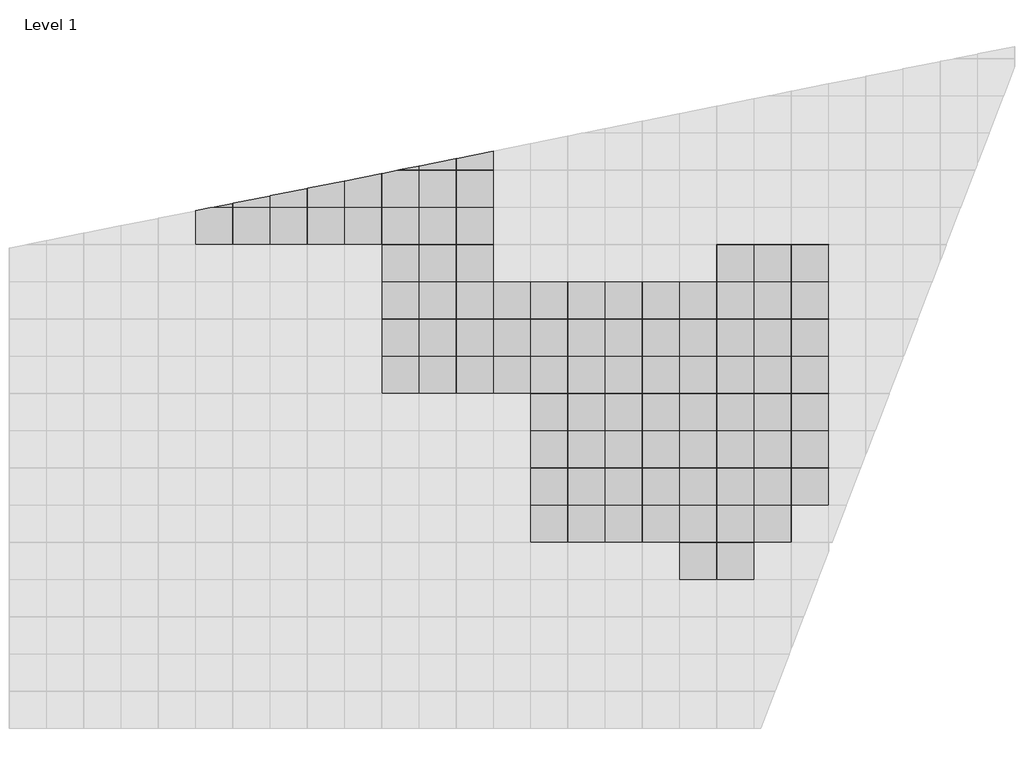
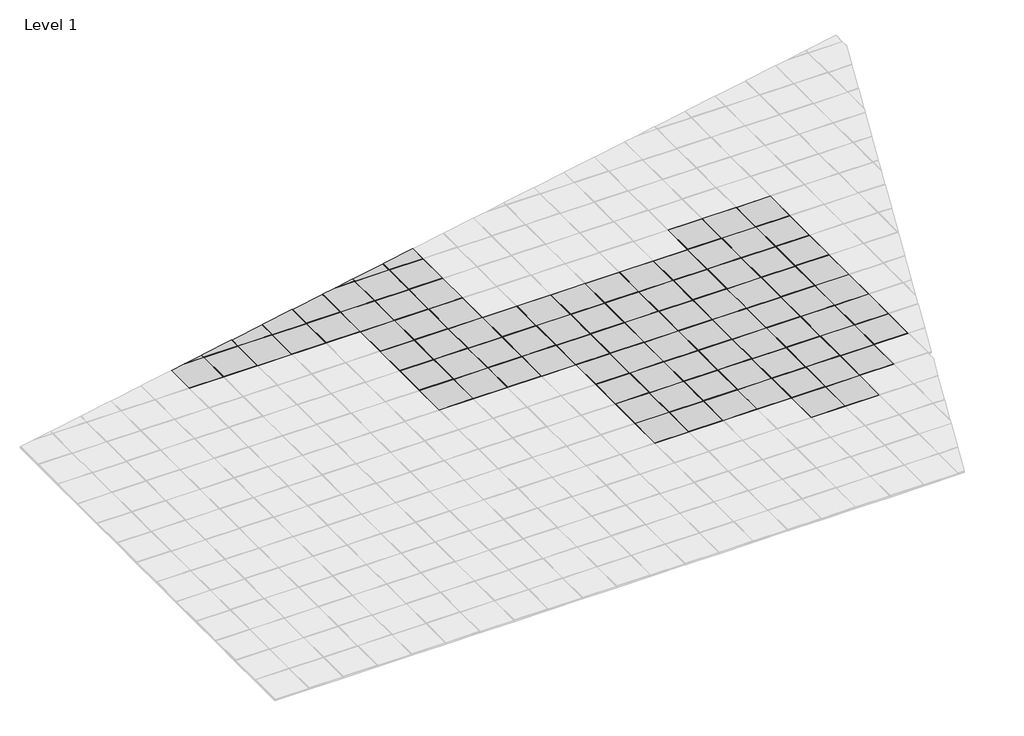
# One storey, part 6 of 18: 94 plates.
"""IFC4 building model written with IfcOpenShell, lengths in millimetres."""

import ifcopenshell
import ifcopenshell.guid

model = None  # the IFC model being written
_history = None  # IfcOwnerHistory: only IFC2X3 demands one
_inside = {}  # id of a spatial element -> (the spatial element, [elements in it])
_under = {}  # id of a project, library or spatial element -> (it, [spatial elements below it])
_declared = {}  # id of a project -> (the project, [libraries it declares])
_typed = {}  # id of a type object -> (the type object, [elements of that type])
_made_of = {}  # id of a material, layer set ... -> (it, [elements and type objects made of it])


def new_model(schema):
    """Start an empty IFC model of exactly this schema.

    Asked for "IFC4X3", IfcOpenShell would pick the latest addendum, in which some entities
    have other attributes; the version numbers below select the first issue.
    IFC2X3 requires an IfcOwnerHistory on every rooted entity: one is made here for all.
    """
    global model, _history
    if schema == "IFC4X3":
        model = ifcopenshell.file(schema_version=(4, 3, 0, 0))
    else:
        model = ifcopenshell.file(schema=schema)
    _inside.clear()
    _under.clear()
    _declared.clear()
    _typed.clear()
    _made_of.clear()
    _history = None
    if model.schema == "IFC2X3":
        org = make("IfcOrganization", Name="unknown")
        user = make(
            "IfcPersonAndOrganization",
            ThePerson=make("IfcPerson", FamilyName="unknown"),
            TheOrganization=org,
        )
        app = make(
            "IfcApplication",
            ApplicationDeveloper=org,
            Version="unknown",
            ApplicationFullName="unknown",
            ApplicationIdentifier="unknown",
        )
        _history = make(
            "IfcOwnerHistory",
            OwningUser=user,
            OwningApplication=app,
            ChangeAction="ADDED",
            CreationDate=0,
        )
    return model


def make(cls, **values):
    """One entity of the class cls with the attributes given. An attribute that is None is left unset."""
    return model.create_entity(
        cls, **{name: value for name, value in values.items() if value is not None}
    )


def rooted(cls, **values):
    """An entity with a GlobalId (a new one), such as an element, a storey or a relation."""
    return make(cls, GlobalId=ifcopenshell.guid.new(), OwnerHistory=_history, **values)


def si_unit(unit_type, name, prefix=None):
    """IfcSIUnit, for example si_unit("LENGTHUNIT", "METRE", prefix="MILLI")."""
    return make("IfcSIUnit", UnitType=unit_type, Prefix=prefix, Name=name)


def assignment(units):
    """IfcUnitAssignment: the units of a project."""
    return None if units is None else make("IfcUnitAssignment", Units=units)


def point(xyz):
    """IfcCartesianPoint."""
    return None if xyz is None else make("IfcCartesianPoint", Coordinates=xyz)


def direction(xyz):
    """IfcDirection."""
    return None if xyz is None else make("IfcDirection", DirectionRatios=xyz)


def frame(location, z_axis=None, x_axis=None):
    """IfcAxis2Placement3D, a coordinate frame: its origin and axes. An axis left out is left unset."""
    return make(
        "IfcAxis2Placement3D",
        Location=point(location),
        Axis=direction(z_axis),
        RefDirection=direction(x_axis),
    )


def origin():
    """The frame at (0, 0, 0) with its axes left unset."""
    return frame((0.0, 0.0, 0.0))


def origin_with_axes():
    """The frame at (0, 0, 0) with the z axis (0, 0, 1) and the x axis (1, 0, 0) written out."""
    return frame((0.0, 0.0, 0.0), z_axis=(0.0, 0.0, 1.0), x_axis=(1.0, 0.0, 0.0))


def place(relative_to, where):
    """IfcLocalPlacement: puts the frame where relative to a parent placement (None: the world)."""
    return make(
        "IfcLocalPlacement", PlacementRelTo=relative_to, RelativePlacement=where
    )


def context(
    kind, dimensions, precision=None, world=None, true_north=None, identifier=None
):
    """IfcGeometricRepresentationContext, for example the 3D "Model" context."""
    return make(
        "IfcGeometricRepresentationContext",
        ContextIdentifier=identifier,
        ContextType=kind,
        CoordinateSpaceDimension=dimensions,
        Precision=precision,
        WorldCoordinateSystem=world,
        TrueNorth=true_north,
    )


def project(units=None, contexts=None):
    """IfcProject with its units and contexts."""
    return rooted(
        "IfcProject",
        Name="project",
        RepresentationContexts=contexts,
        UnitsInContext=assignment(units),
    )


def spatial(cls, under=None, at=None, **own):
    """A site, building, storey or space (cls), placed at a placement, below another one or the project."""
    s = rooted(cls, ObjectPlacement=at, **own)
    if under is not None:
        _under.setdefault(under.id(), (under, []))[1].append(s)
    return s


def polyline(points):
    """IfcPolyline through the points."""
    return make("IfcPolyline", Points=[point(p) for p in points])


def outline(outer, holes=None, kind="AREA"):
    """IfcArbitraryClosedProfileDef: a profile drawn as a closed curve; with holes, ...WithVoids."""
    if holes is None:
        return make("IfcArbitraryClosedProfileDef", ProfileType=kind, OuterCurve=outer)
    return make(
        "IfcArbitraryProfileDefWithVoids",
        ProfileType=kind,
        OuterCurve=outer,
        InnerCurves=holes,
    )


def extrude(swept, where, along, depth):
    """IfcExtrudedAreaSolid: the profile swept, set in the frame where, extruded along a direction by depth."""
    return make(
        "IfcExtrudedAreaSolid",
        SweptArea=swept,
        Position=where,
        ExtrudedDirection=direction(along),
        Depth=depth,
    )


def shape(context_of_items, identifier, shape_type, items):
    """IfcShapeRepresentation: the items that make up one representation, for example the "Body"."""
    return make(
        "IfcShapeRepresentation",
        ContextOfItems=context_of_items,
        RepresentationIdentifier=identifier,
        RepresentationType=shape_type,
        Items=items,
    )


def source(mapping_origin, context_of_items, identifier, shape_type, items):
    """IfcRepresentationMap: a shape defined once, which mapped items show again and again."""
    return make(
        "IfcRepresentationMap",
        MappingOrigin=mapping_origin,
        MappedRepresentation=shape(context_of_items, identifier, shape_type, items),
    )


def transform(
    local_origin,
    x_axis=None,
    y_axis=None,
    z_axis=None,
    scale=None,
    scale2=None,
    scale3=None,
    uniform=True,
):
    """IfcCartesianTransformationOperator3D, or its non-uniform kind. x_axis, y_axis, z_axis: its Axis1, 2, 3."""
    if uniform:
        return make(
            "IfcCartesianTransformationOperator3D",
            Axis1=direction(x_axis),
            Axis2=direction(y_axis),
            LocalOrigin=point(local_origin),
            Scale=scale,
            Axis3=direction(z_axis),
        )
    return make(
        "IfcCartesianTransformationOperator3DnonUniform",
        Axis1=direction(x_axis),
        Axis2=direction(y_axis),
        LocalOrigin=point(local_origin),
        Scale=scale,
        Axis3=direction(z_axis),
        Scale2=scale2,
        Scale3=scale3,
    )


def mapped(mapping_source, mapping_target):
    """IfcMappedItem: shows the shape of a source again, moved by a transform."""
    return make(
        "IfcMappedItem", MappingSource=mapping_source, MappingTarget=mapping_target
    )


def made_of(thing, what):
    """Note that an element or type object is made of a material, layer set ...; save() writes the relation."""
    if what is not None:
        _made_of.setdefault(what.id(), (what, []))[1].append(thing)
    return thing


def element(
    cls,
    number,
    at=None,
    inside=None,
    cuts=None,
    type_object=None,
    material=None,
    context=None,
    identifier="Body",
    shape_type=None,
    held_by="IfcProductDefinitionShape",
    body=None,
    shapes=None,
    **own,
):
    """One element of the class cls, such as IfcWall. Its Tag is "e" and its number.

    at: its placement. inside: the storey or other place that contains it. cuts: it is an
    opening in that element (IfcRelVoidsElement). A single representation is given by context,
    identifier, shape_type and body (its items); several are given by shapes. held_by: the class
    of the entity that holds the representations. save() writes the other relations.
    """
    e = rooted(cls, Tag="e%d" % number, ObjectPlacement=at, **own)
    if body is not None:
        shapes = [shape(context, identifier, shape_type, body)]
    if shapes is not None:
        e.Representation = make(held_by, Representations=shapes)
    if inside is not None:
        _inside.setdefault(inside.id(), (inside, []))[1].append(e)
    if cuts is not None:
        rooted(
            "IfcRelVoidsElement", RelatingBuildingElement=cuts, RelatedOpeningElement=e
        )
    if type_object is not None:
        _typed.setdefault(type_object.id(), (type_object, []))[1].append(e)
    return made_of(e, material)


def aggregate(whole, parts):
    """IfcRelAggregates: a whole, such as a stair, and the parts it consists of."""
    return rooted("IfcRelAggregates", RelatingObject=whole, RelatedObjects=parts)


def save(model, path):
    """Write the relations noted so far, then the file.

    IfcRelAggregates (storeys below a building ...), IfcRelContainedInSpatialStructure (elements
    in a storey), IfcRelDefinesByType, IfcRelAssociatesMaterial and IfcRelDeclares: one each for
    every whole, place, type object, material and project.
    """
    for whole, parts in _under.values():
        aggregate(whole, parts)
    for where, things in _inside.values():
        rooted(
            "IfcRelContainedInSpatialStructure",
            RelatedElements=things,
            RelatingStructure=where,
        )
    for kind, things in _typed.values():
        rooted("IfcRelDefinesByType", RelatedObjects=things, RelatingType=kind)
    for what, things in _made_of.values():
        rooted("IfcRelAssociatesMaterial", RelatedObjects=things, RelatingMaterial=what)
    for by, libraries in _declared.values():
        rooted("IfcRelDeclares", RelatingContext=by, RelatedDefinitions=libraries)
    model.write(path)


def type_1_8eb2385c(model_context):
    return source(origin(), model_context, "Body", "SweptSolid", [
        extrude(outline(polyline([(1000.0, 500.0), (500.0, 500.0), (500.0, 1000.0), (1000.0, 1000.0), (1000.0, 500.0)]), holes=[polyline([(995.0, 995.0), (505.0, 995.0), (505.0, 505.0), (995.0, 505.0), (995.0, 995.0)])]), origin_with_axes(), (0.0, 0.0, 1.0), 18.0),
        extrude(outline(polyline([(505.0, 995.0), (995.0, 995.0), (995.0, 505.0), (505.0, 505.0), (505.0, 995.0)])), origin_with_axes(), (0.0, 0.0, 1.0), 20.0),
    ])


model = new_model("IFC4")

# Units and contexts
model_context = context("Model", 3, world=origin())
ifc_project = project(units=[si_unit("LENGTHUNIT", "METRE", prefix="MILLI")], contexts=[model_context])

# Site, building, storey
site = spatial("IfcSite", under=ifc_project)
building = spatial("IfcBuilding", under=site)
storey = spatial("IfcBuildingStorey", under=building, Name="Level 1", Elevation=0.0)

# Plates
placement = place(None, origin())
element("IfcPlate", 1, ObjectType="00_CPA_tegel : Type 1", at=placement, inside=storey, context=model_context, shape_type="SweptSolid", body=[
    extrude(outline(polyline([(10511.2147669, 19087.7016515), (11001.2147669, 19087.7016515), (11001.2147669, 18597.7016515), (10511.2147669, 18597.7016515), (10511.2147669, 19087.7016515)])), origin_with_axes(), (0.0, 0.0, 1.0), 20.0),
    extrude(outline(polyline([(11006.2147669, 18592.7016515), (10506.2147669, 18592.7016515), (10506.2147669, 19092.7016515), (11006.2147669, 19092.7016515), (11006.2147669, 18592.7016515)]), holes=[polyline([(11001.2147669, 19087.7016515), (10511.2147669, 19087.7016515), (10511.2147669, 18597.7016515), (11001.2147669, 18597.7016515), (11001.2147669, 19087.7016515)])]), origin_with_axes(), (0.0, 0.0, 1.0), 18.0),
])
element("IfcPlate", 2, ObjectType="00_CPA_tegel : Type 1", at=placement, inside=storey, context=model_context, shape_type="SweptSolid", body=[
    extrude(outline(polyline([(14511.2147669, 16587.7016515), (15001.2147669, 16587.7016515), (15001.2147669, 16097.7016515), (14511.2147669, 16097.7016515), (14511.2147669, 16587.7016515)])), origin_with_axes(), (0.0, 0.0, 1.0), 20.0),
    extrude(outline(polyline([(15006.2147669, 16092.7016515), (14506.2147669, 16092.7016515), (14506.2147669, 16592.7016515), (15006.2147669, 16592.7016515), (15006.2147669, 16092.7016515)]), holes=[polyline([(15001.2147669, 16587.7016515), (14511.2147669, 16587.7016515), (14511.2147669, 16097.7016515), (15001.2147669, 16097.7016515), (15001.2147669, 16587.7016515)])]), origin_with_axes(), (0.0, 0.0, 1.0), 18.0),
])
element("IfcPlate", 3, ObjectType="00_CPA_tegel : Type 1", at=placement, inside=storey, context=model_context, shape_type="SweptSolid", body=[
    extrude(outline(polyline([(15011.2147669, 16587.7016515), (15501.2147669, 16587.7016515), (15501.2147669, 16097.7016515), (15011.2147669, 16097.7016515), (15011.2147669, 16587.7016515)])), origin_with_axes(), (0.0, 0.0, 1.0), 20.0),
    extrude(outline(polyline([(15506.2147669, 16092.7016515), (15006.2147669, 16092.7016515), (15006.2147669, 16592.7016515), (15506.2147669, 16592.7016515), (15506.2147669, 16092.7016515)]), holes=[polyline([(15501.2147669, 16587.7016515), (15011.2147669, 16587.7016515), (15011.2147669, 16097.7016515), (15501.2147669, 16097.7016515), (15501.2147669, 16587.7016515)])]), origin_with_axes(), (0.0, 0.0, 1.0), 18.0),
])
element("IfcPlate", 4, ObjectType="00_CPA_tegel : Type 1", at=placement, inside=storey, context=model_context, shape_type="SweptSolid", body=[
    extrude(outline(polyline([(15011.2147669, 17087.7016515), (15501.2147669, 17087.7016515), (15501.2147669, 16597.7016515), (15011.2147669, 16597.7016515), (15011.2147669, 17087.7016515)])), origin_with_axes(), (0.0, 0.0, 1.0), 20.0),
    extrude(outline(polyline([(15506.2147669, 16592.7016515), (15006.2147669, 16592.7016515), (15006.2147669, 17092.7016515), (15506.2147669, 17092.7016515), (15506.2147669, 16592.7016515)]), holes=[polyline([(15501.2147669, 17087.7016515), (15011.2147669, 17087.7016515), (15011.2147669, 16597.7016515), (15501.2147669, 16597.7016515), (15501.2147669, 17087.7016515)])]), origin_with_axes(), (0.0, 0.0, 1.0), 18.0),
])
element("IfcPlate", 5, ObjectType="00_CPA_tegel : Type 1", at=placement, inside=storey, context=model_context, shape_type="SweptSolid", body=[
    extrude(outline(polyline([(10511.2147669, 19587.7016515), (11001.2147669, 19587.7016515), (11001.2147669, 19097.7016515), (10511.2147669, 19097.7016515), (10511.2147669, 19587.7016515)])), origin_with_axes(), (0.0, 0.0, 1.0), 20.0),
    extrude(outline(polyline([(11006.2147669, 19092.7016515), (10506.2147669, 19092.7016515), (10506.2147669, 19592.7016515), (11006.2147669, 19592.7016515), (11006.2147669, 19092.7016515)]), holes=[polyline([(11001.2147669, 19587.7016515), (10511.2147669, 19587.7016515), (10511.2147669, 19097.7016515), (11001.2147669, 19097.7016515), (11001.2147669, 19587.7016515)])]), origin_with_axes(), (0.0, 0.0, 1.0), 18.0),
])
element("IfcPlate", 6, ObjectType="00_CPA_tegel : Type 1", at=placement, inside=storey, context=model_context, shape_type="SweptSolid", body=[
    extrude(outline(polyline([(11011.2147669, 19587.7016515), (11501.2147669, 19587.7016515), (11501.2147669, 19097.7016515), (11011.2147669, 19097.7016515), (11011.2147669, 19587.7016515)])), origin_with_axes(), (0.0, 0.0, 1.0), 20.0),
    extrude(outline(polyline([(11506.2147669, 19092.7016515), (11006.2147669, 19092.7016515), (11006.2147669, 19592.7016515), (11506.2147669, 19592.7016515), (11506.2147669, 19092.7016515)]), holes=[polyline([(11501.2147669, 19587.7016515), (11011.2147669, 19587.7016515), (11011.2147669, 19097.7016515), (11501.2147669, 19097.7016515), (11501.2147669, 19587.7016515)])]), origin_with_axes(), (0.0, 0.0, 1.0), 18.0),
])
element("IfcPlate", 7, ObjectType="00_CPA_tegel : Type 1", at=placement, inside=storey, context=model_context, shape_type="SweptSolid", body=[
    extrude(outline(polyline([(11011.2147669, 20087.7016515), (11501.2147669, 20087.7016515), (11501.2147669, 19597.7016515), (11011.2147669, 19597.7016515), (11011.2147669, 20087.7016515)])), origin_with_axes(), (0.0, 0.0, 1.0), 20.0),
    extrude(outline(polyline([(11506.2147669, 19592.7016515), (11006.2147669, 19592.7016515), (11006.2147669, 20092.7016515), (11506.2147669, 20092.7016515), (11506.2147669, 19592.7016515)]), holes=[polyline([(11501.2147669, 20087.7016515), (11011.2147669, 20087.7016515), (11011.2147669, 19597.7016515), (11501.2147669, 19597.7016515), (11501.2147669, 20087.7016515)])]), origin_with_axes(), (0.0, 0.0, 1.0), 18.0),
])
element("IfcPlate", 8, ObjectType="00_CPA_tegel : Type 1", at=placement, inside=storey, context=model_context, shape_type="SweptSolid", body=[
    extrude(outline(polyline([(11511.2147669, 20087.7016515), (12001.2147669, 20087.7016515), (12001.2147669, 19597.7016515), (11511.2147669, 19597.7016515), (11511.2147669, 20087.7016515)])), origin_with_axes(), (0.0, 0.0, 1.0), 20.0),
    extrude(outline(polyline([(12006.2147669, 19592.7016515), (11506.2147669, 19592.7016515), (11506.2147669, 20092.7016515), (12006.2147669, 20092.7016515), (12006.2147669, 19592.7016515)]), holes=[polyline([(12001.2147669, 20087.7016515), (11511.2147669, 20087.7016515), (11511.2147669, 19597.7016515), (12001.2147669, 19597.7016515), (12001.2147669, 20087.7016515)])]), origin_with_axes(), (0.0, 0.0, 1.0), 18.0),
])
element("IfcPlate", 9, ObjectType="00_CPA_tegel : Type 1", at=placement, inside=storey, context=model_context, shape_type="SweptSolid", body=[
    extrude(outline(polyline([(12011.2147669, 20087.7016515), (12501.2147669, 20087.7016515), (12501.2147669, 19597.7016515), (12011.2147669, 19597.7016515), (12011.2147669, 20087.7016515)])), origin_with_axes(), (0.0, 0.0, 1.0), 20.0),
    extrude(outline(polyline([(12506.2147669, 19592.7016515), (12006.2147669, 19592.7016515), (12006.2147669, 20092.7016515), (12506.2147669, 20092.7016515), (12506.2147669, 19592.7016515)]), holes=[polyline([(12501.2147669, 20087.7016515), (12011.2147669, 20087.7016515), (12011.2147669, 19597.7016515), (12501.2147669, 19597.7016515), (12501.2147669, 20087.7016515)])]), origin_with_axes(), (0.0, 0.0, 1.0), 18.0),
])
element("IfcPlate", 10, ObjectType="00_CPA_tegel : Type 1", at=placement, inside=storey, context=model_context, shape_type="SweptSolid", body=[
    extrude(outline(polyline([(12511.2147669, 20087.7016515), (13001.2147669, 20087.7016515), (13001.2147669, 19597.7016515), (12511.2147669, 19597.7016515), (12511.2147669, 20087.7016515)])), origin_with_axes(), (0.0, 0.0, 1.0), 20.0),
    extrude(outline(polyline([(13006.2147669, 19592.7016515), (12506.2147669, 19592.7016515), (12506.2147669, 20092.7016515), (13006.2147669, 20092.7016515), (13006.2147669, 19592.7016515)]), holes=[polyline([(13001.2147669, 20087.7016515), (12511.2147669, 20087.7016515), (12511.2147669, 19597.7016515), (13001.2147669, 19597.7016515), (13001.2147669, 20087.7016515)])]), origin_with_axes(), (0.0, 0.0, 1.0), 18.0),
])
element("IfcPlate", 11, ObjectType="00_CPA_tegel : Type 1", at=placement, inside=storey, context=model_context, shape_type="SweptSolid", body=[
    extrude(outline(polyline([(13011.2147669, 20087.7016515), (13501.2147669, 20087.7016515), (13501.2147669, 19597.7016515), (13011.2147669, 19597.7016515), (13011.2147669, 20087.7016515)])), origin_with_axes(), (0.0, 0.0, 1.0), 20.0),
    extrude(outline(polyline([(13506.2147669, 19592.7016515), (13006.2147669, 19592.7016515), (13006.2147669, 20092.7016515), (13506.2147669, 20092.7016515), (13506.2147669, 19592.7016515)]), holes=[polyline([(13501.2147669, 20087.7016515), (13011.2147669, 20087.7016515), (13011.2147669, 19597.7016515), (13501.2147669, 19597.7016515), (13501.2147669, 20087.7016515)])]), origin_with_axes(), (0.0, 0.0, 1.0), 18.0),
])
element("IfcPlate", 12, ObjectType="00_CPA_tegel : Type 1", at=placement, inside=storey, context=model_context, shape_type="SweptSolid", body=[
    extrude(outline(polyline([(11011.2147669, 20587.7016515), (11501.2147669, 20587.7016515), (11501.2147669, 20097.7016515), (11011.2147669, 20097.7016515), (11011.2147669, 20587.7016515)])), origin_with_axes(), (0.0, 0.0, 1.0), 20.0),
    extrude(outline(polyline([(11506.2147669, 20092.7016515), (11006.2147669, 20092.7016515), (11006.2147669, 20592.7016515), (11506.2147669, 20592.7016515), (11506.2147669, 20092.7016515)]), holes=[polyline([(11501.2147669, 20587.7016515), (11011.2147669, 20587.7016515), (11011.2147669, 20097.7016515), (11501.2147669, 20097.7016515), (11501.2147669, 20587.7016515)])]), origin_with_axes(), (0.0, 0.0, 1.0), 18.0),
])
element("IfcPlate", 13, ObjectType="00_CPA_tegel : Type 1", at=placement, inside=storey, context=model_context, shape_type="SweptSolid", body=[
    extrude(outline(polyline([(11511.2147669, 20587.7016515), (12001.2147669, 20587.7016515), (12001.2147669, 20097.7016515), (11511.2147669, 20097.7016515), (11511.2147669, 20587.7016515)])), origin_with_axes(), (0.0, 0.0, 1.0), 20.0),
    extrude(outline(polyline([(12006.2147669, 20092.7016515), (11506.2147669, 20092.7016515), (11506.2147669, 20592.7016515), (12006.2147669, 20592.7016515), (12006.2147669, 20092.7016515)]), holes=[polyline([(12001.2147669, 20587.7016515), (11511.2147669, 20587.7016515), (11511.2147669, 20097.7016515), (12001.2147669, 20097.7016515), (12001.2147669, 20587.7016515)])]), origin_with_axes(), (0.0, 0.0, 1.0), 18.0),
])
element("IfcPlate", 14, ObjectType="00_CPA_tegel : Type 1", at=placement, inside=storey, context=model_context, shape_type="SweptSolid", body=[
    extrude(outline(polyline([(8501.2147669, 20597.7016515), (8011.2147669, 20597.7016515), (8011.2147669, 21048.3944739), (8207.0466363, 21087.7016515), (8501.2147669, 21087.7016515), (8501.2147669, 20597.7016515)])), origin_with_axes(), (0.0, 0.0, 1.0), 20.0),
    extrude(outline(polyline([(8506.2147669, 20592.7016515), (8006.2147669, 20592.7016515), (8006.2147669, 21047.3908788), (8011.2147669, 21048.3944739), (8011.2147669, 20597.7016515), (8501.2147669, 20597.7016515), (8501.2147669, 21087.7016515), (8207.0466363, 21087.7016515), (8231.9570828, 21092.7016515), (8506.2147669, 21092.7016515), (8506.2147669, 20592.7016515)])), origin_with_axes(), (0.0, 0.0, 1.0), 18.0),
])
element("IfcPlate", 15, ObjectType="00_CPA_tegel : Type 1", at=placement, inside=storey, context=model_context, shape_type="SweptSolid", body=[
    extrude(outline(polyline([(11511.2147669, 21087.7016515), (12001.2147669, 21087.7016515), (12001.2147669, 20597.7016515), (11511.2147669, 20597.7016515), (11511.2147669, 21087.7016515)])), origin_with_axes(), (0.0, 0.0, 1.0), 20.0),
    extrude(outline(polyline([(12006.2147669, 20592.7016515), (11506.2147669, 20592.7016515), (11506.2147669, 21092.7016515), (12006.2147669, 21092.7016515), (12006.2147669, 20592.7016515)]), holes=[polyline([(12001.2147669, 21087.7016515), (11511.2147669, 21087.7016515), (11511.2147669, 20597.7016515), (12001.2147669, 20597.7016515), (12001.2147669, 21087.7016515)])]), origin_with_axes(), (0.0, 0.0, 1.0), 18.0),
])
element("IfcPlate", 16, ObjectType="00_CPA_tegel : Type 1", at=placement, inside=storey, context=model_context, shape_type="SweptSolid", body=[
    extrude(outline(polyline([(8501.2147669, 21097.7016515), (8256.8675294, 21097.7016515), (8501.2147669, 21146.7467855), (8501.2147669, 21097.7016515)])), origin_with_axes(), (0.0, 0.0, 1.0), 20.0),
    extrude(outline(polyline([(8506.2147669, 21092.7016515), (8231.9570828, 21092.7016515), (8256.8675294, 21097.7016515), (8501.2147669, 21097.7016515), (8501.2147669, 21146.7467855), (8506.2147669, 21147.7503805), (8506.2147669, 21092.7016515)])), origin_with_axes(), (0.0, 0.0, 1.0), 18.0),
])
element("IfcPlate", 17, ObjectType="00_CPA_tegel : Type 1", at=placement, inside=storey, context=model_context, shape_type="SweptSolid", body=[
    extrude(outline(polyline([(9001.2147669, 21097.7016515), (8511.2147669, 21097.7016515), (8511.2147669, 21148.7539755), (9001.2147669, 21247.1062872), (9001.2147669, 21097.7016515)])), origin_with_axes(), (0.0, 0.0, 1.0), 20.0),
    extrude(outline(polyline([(9006.2147669, 21092.7016515), (8506.2147669, 21092.7016515), (8506.2147669, 21147.7503805), (8511.2147669, 21148.7539755), (8511.2147669, 21097.7016515), (9001.2147669, 21097.7016515), (9001.2147669, 21247.1062872), (9006.2147669, 21248.1098822), (9006.2147669, 21092.7016515)])), origin_with_axes(), (0.0, 0.0, 1.0), 18.0),
])
element("IfcPlate", 18, ObjectType="00_CPA_tegel : Type 1", at=placement, inside=storey, context=model_context, shape_type="SweptSolid", body=[
    extrude(outline(polyline([(9501.2147669, 21097.7016515), (9011.2147669, 21097.7016515), (9011.2147669, 21249.1134772), (9501.2147669, 21347.4657889), (9501.2147669, 21097.7016515)])), origin_with_axes(), (0.0, 0.0, 1.0), 20.0),
    extrude(outline(polyline([(9506.2147669, 21092.7016515), (9006.2147669, 21092.7016515), (9006.2147669, 21248.1098822), (9011.2147669, 21249.1134772), (9011.2147669, 21097.7016515), (9501.2147669, 21097.7016515), (9501.2147669, 21347.4657889), (9506.2147669, 21348.4693839), (9506.2147669, 21092.7016515)])), origin_with_axes(), (0.0, 0.0, 1.0), 18.0),
])
element("IfcPlate", 19, ObjectType="00_CPA_tegel : Type 1", at=placement, inside=storey, context=model_context, shape_type="SweptSolid", body=[
    extrude(outline(polyline([(10001.2147669, 21097.7016515), (9511.2147669, 21097.7016515), (9511.2147669, 21349.4729789), (10001.2147669, 21447.8252906), (10001.2147669, 21097.7016515)])), origin_with_axes(), (0.0, 0.0, 1.0), 20.0),
    extrude(outline(polyline([(10006.2147669, 21092.7016515), (9506.2147669, 21092.7016515), (9506.2147669, 21348.4693839), (9511.2147669, 21349.4729789), (9511.2147669, 21097.7016515), (10001.2147669, 21097.7016515), (10001.2147669, 21447.8252906), (10006.2147669, 21448.8288856), (10006.2147669, 21092.7016515)])), origin_with_axes(), (0.0, 0.0, 1.0), 18.0),
])
element("IfcPlate", 20, ObjectType="00_CPA_tegel : Type 1", at=placement, inside=storey, context=model_context, shape_type="SweptSolid", body=[
    extrude(outline(polyline([(10501.2147669, 21097.7016515), (10011.2147669, 21097.7016515), (10011.2147669, 21449.8324806), (10501.2147669, 21548.1847922), (10501.2147669, 21097.7016515)])), origin_with_axes(), (0.0, 0.0, 1.0), 20.0),
    extrude(outline(polyline([(10506.2147669, 21092.7016515), (10006.2147669, 21092.7016515), (10006.2147669, 21448.8288856), (10011.2147669, 21449.8324806), (10011.2147669, 21097.7016515), (10501.2147669, 21097.7016515), (10501.2147669, 21548.1847922), (10506.2147669, 21549.1883873), (10506.2147669, 21092.7016515)])), origin_with_axes(), (0.0, 0.0, 1.0), 18.0),
])
element("IfcPlate", 21, ObjectType="00_CPA_tegel : Type 1", at=placement, inside=storey, context=model_context, shape_type="SweptSolid", body=[
    extrude(outline(polyline([(11001.2147669, 21097.7016515), (10511.2147669, 21097.7016515), (10511.2147669, 21550.1919823), (10698.0912888, 21587.7016515), (11001.2147669, 21587.7016515), (11001.2147669, 21097.7016515)])), origin_with_axes(), (0.0, 0.0, 1.0), 20.0),
    extrude(outline(polyline([(11006.2147669, 21092.7016515), (10506.2147669, 21092.7016515), (10506.2147669, 21549.1883873), (10511.2147669, 21550.1919823), (10511.2147669, 21097.7016515), (11001.2147669, 21097.7016515), (11001.2147669, 21587.7016515), (10698.0912888, 21587.7016515), (10723.0017353, 21592.7016515), (11006.2147669, 21592.7016515), (11006.2147669, 21092.7016515)])), origin_with_axes(), (0.0, 0.0, 1.0), 18.0),
])
element("IfcPlate", 22, ObjectType="00_CPA_tegel : Type 1", at=placement, inside=storey, context=model_context, shape_type="SweptSolid", body=[
    extrude(outline(polyline([(11511.2147669, 21587.7016515), (12001.2147669, 21587.7016515), (12001.2147669, 21097.7016515), (11511.2147669, 21097.7016515), (11511.2147669, 21587.7016515)])), origin_with_axes(), (0.0, 0.0, 1.0), 20.0),
    extrude(outline(polyline([(12006.2147669, 21092.7016515), (11506.2147669, 21092.7016515), (11506.2147669, 21592.7016515), (12006.2147669, 21592.7016515), (12006.2147669, 21092.7016515)]), holes=[polyline([(12001.2147669, 21587.7016515), (11511.2147669, 21587.7016515), (11511.2147669, 21097.7016515), (12001.2147669, 21097.7016515), (12001.2147669, 21587.7016515)])]), origin_with_axes(), (0.0, 0.0, 1.0), 18.0),
])
element("IfcPlate", 23, ObjectType="00_CPA_tegel : Type 1", at=placement, inside=storey, context=model_context, shape_type="SweptSolid", body=[
    extrude(outline(polyline([(11001.2147669, 21597.7016515), (10747.9121819, 21597.7016515), (11001.2147669, 21648.5442939), (11001.2147669, 21597.7016515)])), origin_with_axes(), (0.0, 0.0, 1.0), 20.0),
    extrude(outline(polyline([(11006.2147669, 21592.7016515), (10723.0017353, 21592.7016515), (10747.9121819, 21597.7016515), (11001.2147669, 21597.7016515), (11001.2147669, 21648.5442939), (11006.2147669, 21649.5478889), (11006.2147669, 21592.7016515)])), origin_with_axes(), (0.0, 0.0, 1.0), 18.0),
])
element("IfcPlate", 24, ObjectType="00_CPA_tegel : Type 1", at=placement, inside=storey, context=model_context, shape_type="SweptSolid", body=[
    extrude(outline(polyline([(11501.2147669, 21597.7016515), (11011.2147669, 21597.7016515), (11011.2147669, 21650.551484), (11501.2147669, 21748.9037956), (11501.2147669, 21597.7016515)])), origin_with_axes(), (0.0, 0.0, 1.0), 20.0),
    extrude(outline(polyline([(11506.2147669, 21592.7016515), (11006.2147669, 21592.7016515), (11006.2147669, 21649.5478889), (11011.2147669, 21650.551484), (11011.2147669, 21597.7016515), (11501.2147669, 21597.7016515), (11501.2147669, 21748.9037956), (11506.2147669, 21749.9073906), (11506.2147669, 21592.7016515)])), origin_with_axes(), (0.0, 0.0, 1.0), 18.0),
])
element("IfcPlate", 25, ObjectType="00_CPA_tegel : Type 1", at=placement, inside=storey, context=model_context, shape_type="SweptSolid", body=[
    extrude(outline(polyline([(12001.2147669, 21597.7016515), (11511.2147669, 21597.7016515), (11511.2147669, 21750.9109856), (12001.2147669, 21849.2632973), (12001.2147669, 21597.7016515)])), origin_with_axes(), (0.0, 0.0, 1.0), 20.0),
    extrude(outline(polyline([(12006.2147669, 21592.7016515), (11506.2147669, 21592.7016515), (11506.2147669, 21749.9073906), (11511.2147669, 21750.9109856), (11511.2147669, 21597.7016515), (12001.2147669, 21597.7016515), (12001.2147669, 21849.2632973), (12006.2147669, 21850.2668923), (12006.2147669, 21592.7016515)])), origin_with_axes(), (0.0, 0.0, 1.0), 18.0),
])
type_1_shape = type_1_8eb2385c(model_context)
element("IfcPlate", 26, ObjectType="00_CPA_tegel : Type 1", at=placement, inside=storey, context=model_context, shape_type="MappedRepresentation", body=[
    mapped(type_1_shape, transform((10506.2147669, 18092.7016515, 0.0), x_axis=(1.0000000000000002, 0.0, 0.0), y_axis=(0.0, 1.0000000000000002, 0.0), z_axis=(0.0, 0.0, 1.0))),
])
element("IfcPlate", 27, ObjectType="00_CPA_tegel : Type 1", at=placement, inside=storey, context=model_context, shape_type="MappedRepresentation", body=[
    mapped(type_1_shape, transform((11006.2147669, 18092.7016515, 0.0), x_axis=(1.0000000000000002, 0.0, 0.0), y_axis=(0.0, 1.0000000000000002, 0.0), z_axis=(0.0, 0.0, 1.0))),
])
element("IfcPlate", 28, ObjectType="00_CPA_tegel : Type 1", at=placement, inside=storey, context=model_context, shape_type="MappedRepresentation", body=[
    mapped(type_1_shape, transform((11506.2147669, 18092.7016515, 0.0), x_axis=(1.0000000000000002, 0.0, 0.0), y_axis=(0.0, 1.0000000000000002, 0.0), z_axis=(0.0, 0.0, 1.0))),
])
element("IfcPlate", 29, ObjectType="00_CPA_tegel : Type 1", at=placement, inside=storey, context=model_context, shape_type="MappedRepresentation", body=[
    mapped(type_1_shape, transform((12006.2147669, 16092.7016515, 0.0), x_axis=(1.0000000000000002, 0.0, 0.0), y_axis=(0.0, 1.0000000000000002, 0.0), z_axis=(0.0, 0.0, 1.0))),
])
element("IfcPlate", 30, ObjectType="00_CPA_tegel : Type 1", at=placement, inside=storey, context=model_context, shape_type="MappedRepresentation", body=[
    mapped(type_1_shape, transform((12506.2147669, 16092.7016515, 0.0), x_axis=(1.0000000000000002, 0.0, 0.0), y_axis=(0.0, 1.0000000000000002, 0.0), z_axis=(0.0, 0.0, 1.0))),
])
element("IfcPlate", 31, ObjectType="00_CPA_tegel : Type 1", at=placement, inside=storey, context=model_context, shape_type="MappedRepresentation", body=[
    mapped(type_1_shape, transform((13006.2147669, 16092.7016515, 0.0), x_axis=(1.0000000000000002, 0.0, 0.0), y_axis=(0.0, 1.0000000000000002, 0.0), z_axis=(0.0, 0.0, 1.0))),
])
element("IfcPlate", 32, ObjectType="00_CPA_tegel : Type 1", at=placement, inside=storey, context=model_context, shape_type="MappedRepresentation", body=[
    mapped(type_1_shape, transform((13506.2147669, 16092.7016515, 0.0), x_axis=(1.0000000000000002, 0.0, 0.0), y_axis=(0.0, 1.0000000000000002, 0.0), z_axis=(0.0, 0.0, 1.0))),
])
element("IfcPlate", 33, ObjectType="00_CPA_tegel : Type 1", at=placement, inside=storey, context=model_context, shape_type="MappedRepresentation", body=[
    mapped(type_1_shape, transform((14006.2147669, 16092.7016515, 0.0), x_axis=(1.0000000000000002, 0.0, 0.0), y_axis=(0.0, 1.0000000000000002, 0.0), z_axis=(0.0, 0.0, 1.0))),
])
element("IfcPlate", 34, ObjectType="00_CPA_tegel : Type 1", at=placement, inside=storey, context=model_context, shape_type="MappedRepresentation", body=[
    mapped(type_1_shape, transform((15006.2147669, 16092.7016515, 0.0), x_axis=(1.0000000000000002, 0.0, 0.0), y_axis=(0.0, 1.0000000000000002, 0.0), z_axis=(0.0, 0.0, 1.0))),
])
element("IfcPlate", 35, ObjectType="00_CPA_tegel : Type 1", at=placement, inside=storey, context=model_context, shape_type="MappedRepresentation", body=[
    mapped(type_1_shape, transform((12006.2147669, 16592.7016515, 0.0), x_axis=(1.0000000000000002, 0.0, 0.0), y_axis=(0.0, 1.0000000000000002, 0.0), z_axis=(0.0, 0.0, 1.0))),
])
element("IfcPlate", 36, ObjectType="00_CPA_tegel : Type 1", at=placement, inside=storey, context=model_context, shape_type="MappedRepresentation", body=[
    mapped(type_1_shape, transform((12506.2147669, 16592.7016515, 0.0), x_axis=(1.0000000000000002, 0.0, 0.0), y_axis=(0.0, 1.0000000000000002, 0.0), z_axis=(0.0, 0.0, 1.0))),
])
element("IfcPlate", 37, ObjectType="00_CPA_tegel : Type 1", at=placement, inside=storey, context=model_context, shape_type="MappedRepresentation", body=[
    mapped(type_1_shape, transform((13006.2147669, 16592.7016515, 0.0), x_axis=(1.0000000000000002, 0.0, 0.0), y_axis=(0.0, 1.0000000000000002, 0.0), z_axis=(0.0, 0.0, 1.0))),
])
element("IfcPlate", 38, ObjectType="00_CPA_tegel : Type 1", at=placement, inside=storey, context=model_context, shape_type="MappedRepresentation", body=[
    mapped(type_1_shape, transform((13506.2147669, 16592.7016515, 0.0), x_axis=(1.0000000000000002, 0.0, 0.0), y_axis=(0.0, 1.0000000000000002, 0.0), z_axis=(0.0, 0.0, 1.0))),
])
element("IfcPlate", 39, ObjectType="00_CPA_tegel : Type 1", at=placement, inside=storey, context=model_context, shape_type="MappedRepresentation", body=[
    mapped(type_1_shape, transform((14006.2147669, 16592.7016515, 0.0), x_axis=(1.0000000000000002, 0.0, 0.0), y_axis=(0.0, 1.0000000000000002, 0.0), z_axis=(0.0, 0.0, 1.0))),
])
element("IfcPlate", 40, ObjectType="00_CPA_tegel : Type 1", at=placement, inside=storey, context=model_context, shape_type="MappedRepresentation", body=[
    mapped(type_1_shape, transform((14506.2147669, 16592.7016515, 0.0), x_axis=(1.0000000000000002, 0.0, 0.0), y_axis=(0.0, 1.0000000000000002, 0.0), z_axis=(0.0, 0.0, 1.0))),
])
element("IfcPlate", 41, ObjectType="00_CPA_tegel : Type 1", at=placement, inside=storey, context=model_context, shape_type="MappedRepresentation", body=[
    mapped(type_1_shape, transform((15006.2147669, 16592.7016515, 0.0), x_axis=(1.0000000000000002, 0.0, 0.0), y_axis=(0.0, 1.0000000000000002, 0.0), z_axis=(0.0, 0.0, 1.0))),
])
element("IfcPlate", 42, ObjectType="00_CPA_tegel : Type 1", at=placement, inside=storey, context=model_context, shape_type="MappedRepresentation", body=[
    mapped(type_1_shape, transform((15506.2147669, 16592.7016515, 0.0), x_axis=(1.0000000000000002, 0.0, 0.0), y_axis=(0.0, 1.0000000000000002, 0.0), z_axis=(0.0, 0.0, 1.0))),
])
element("IfcPlate", 43, ObjectType="00_CPA_tegel : Type 1", at=placement, inside=storey, context=model_context, shape_type="MappedRepresentation", body=[
    mapped(type_1_shape, transform((12006.2147669, 17092.7016515, 0.0), x_axis=(1.0000000000000002, 0.0, 0.0), y_axis=(0.0, 1.0000000000000002, 0.0), z_axis=(0.0, 0.0, 1.0))),
])
element("IfcPlate", 44, ObjectType="00_CPA_tegel : Type 1", at=placement, inside=storey, context=model_context, shape_type="MappedRepresentation", body=[
    mapped(type_1_shape, transform((12506.2147669, 17092.7016515, 0.0), x_axis=(1.0000000000000002, 0.0, 0.0), y_axis=(0.0, 1.0000000000000002, 0.0), z_axis=(0.0, 0.0, 1.0))),
])
element("IfcPlate", 45, ObjectType="00_CPA_tegel : Type 1", at=placement, inside=storey, context=model_context, shape_type="MappedRepresentation", body=[
    mapped(type_1_shape, transform((13006.2147669, 17092.7016515, 0.0), x_axis=(1.0000000000000002, 0.0, 0.0), y_axis=(0.0, 1.0000000000000002, 0.0), z_axis=(0.0, 0.0, 1.0))),
])
element("IfcPlate", 46, ObjectType="00_CPA_tegel : Type 1", at=placement, inside=storey, context=model_context, shape_type="MappedRepresentation", body=[
    mapped(type_1_shape, transform((13506.2147669, 17092.7016515, 0.0), x_axis=(1.0000000000000002, 0.0, 0.0), y_axis=(0.0, 1.0000000000000002, 0.0), z_axis=(0.0, 0.0, 1.0))),
])
element("IfcPlate", 47, ObjectType="00_CPA_tegel : Type 1", at=placement, inside=storey, context=model_context, shape_type="MappedRepresentation", body=[
    mapped(type_1_shape, transform((14006.2147669, 17092.7016515, 0.0), x_axis=(1.0000000000000002, 0.0, 0.0), y_axis=(0.0, 1.0000000000000002, 0.0), z_axis=(0.0, 0.0, 1.0))),
])
element("IfcPlate", 48, ObjectType="00_CPA_tegel : Type 1", at=placement, inside=storey, context=model_context, shape_type="MappedRepresentation", body=[
    mapped(type_1_shape, transform((14506.2147669, 17092.7016515, 0.0), x_axis=(1.0000000000000002, 0.0, 0.0), y_axis=(0.0, 1.0000000000000002, 0.0), z_axis=(0.0, 0.0, 1.0))),
])
element("IfcPlate", 49, ObjectType="00_CPA_tegel : Type 1", at=placement, inside=storey, context=model_context, shape_type="MappedRepresentation", body=[
    mapped(type_1_shape, transform((15006.2147669, 17092.7016515, 0.0), x_axis=(1.0000000000000002, 0.0, 0.0), y_axis=(0.0, 1.0000000000000002, 0.0), z_axis=(0.0, 0.0, 1.0))),
])
element("IfcPlate", 50, ObjectType="00_CPA_tegel : Type 1", at=placement, inside=storey, context=model_context, shape_type="MappedRepresentation", body=[
    mapped(type_1_shape, transform((15506.2147669, 17092.7016515, 0.0), x_axis=(1.0000000000000002, 0.0, 0.0), y_axis=(0.0, 1.0000000000000002, 0.0), z_axis=(0.0, 0.0, 1.0))),
])
element("IfcPlate", 51, ObjectType="00_CPA_tegel : Type 1", at=placement, inside=storey, context=model_context, shape_type="MappedRepresentation", body=[
    mapped(type_1_shape, transform((12006.2147669, 17592.7016515, 0.0), x_axis=(1.0000000000000002, 0.0, 0.0), y_axis=(0.0, 1.0000000000000002, 0.0), z_axis=(0.0, 0.0, 1.0))),
])
element("IfcPlate", 52, ObjectType="00_CPA_tegel : Type 1", at=placement, inside=storey, context=model_context, shape_type="MappedRepresentation", body=[
    mapped(type_1_shape, transform((12506.2147669, 17592.7016515, 0.0), x_axis=(1.0000000000000002, 0.0, 0.0), y_axis=(0.0, 1.0000000000000002, 0.0), z_axis=(0.0, 0.0, 1.0))),
])
element("IfcPlate", 53, ObjectType="00_CPA_tegel : Type 1", at=placement, inside=storey, context=model_context, shape_type="MappedRepresentation", body=[
    mapped(type_1_shape, transform((13006.2147669, 17592.7016515, 0.0), x_axis=(1.0000000000000002, 0.0, 0.0), y_axis=(0.0, 1.0000000000000002, 0.0), z_axis=(0.0, 0.0, 1.0))),
])
element("IfcPlate", 54, ObjectType="00_CPA_tegel : Type 1", at=placement, inside=storey, context=model_context, shape_type="MappedRepresentation", body=[
    mapped(type_1_shape, transform((13506.2147669, 17592.7016515, 0.0), x_axis=(1.0000000000000002, 0.0, 0.0), y_axis=(0.0, 1.0000000000000002, 0.0), z_axis=(0.0, 0.0, 1.0))),
])
element("IfcPlate", 55, ObjectType="00_CPA_tegel : Type 1", at=placement, inside=storey, context=model_context, shape_type="MappedRepresentation", body=[
    mapped(type_1_shape, transform((14006.2147669, 17592.7016515, 0.0), x_axis=(1.0000000000000002, 0.0, 0.0), y_axis=(0.0, 1.0000000000000002, 0.0), z_axis=(0.0, 0.0, 1.0))),
])
element("IfcPlate", 56, ObjectType="00_CPA_tegel : Type 1", at=placement, inside=storey, context=model_context, shape_type="MappedRepresentation", body=[
    mapped(type_1_shape, transform((14506.2147669, 17592.7016515, 0.0), x_axis=(1.0000000000000002, 0.0, 0.0), y_axis=(0.0, 1.0000000000000002, 0.0), z_axis=(0.0, 0.0, 1.0))),
])
element("IfcPlate", 57, ObjectType="00_CPA_tegel : Type 1", at=placement, inside=storey, context=model_context, shape_type="MappedRepresentation", body=[
    mapped(type_1_shape, transform((15006.2147669, 17592.7016515, 0.0), x_axis=(1.0000000000000002, 0.0, 0.0), y_axis=(0.0, 1.0000000000000002, 0.0), z_axis=(0.0, 0.0, 1.0))),
])
element("IfcPlate", 58, ObjectType="00_CPA_tegel : Type 1", at=placement, inside=storey, context=model_context, shape_type="MappedRepresentation", body=[
    mapped(type_1_shape, transform((15506.2147669, 17592.7016515, 0.0), x_axis=(1.0000000000000002, 0.0, 0.0), y_axis=(0.0, 1.0000000000000002, 0.0), z_axis=(0.0, 0.0, 1.0))),
])
element("IfcPlate", 59, ObjectType="00_CPA_tegel : Type 1", at=placement, inside=storey, context=model_context, shape_type="MappedRepresentation", body=[
    mapped(type_1_shape, transform((12006.2147669, 18092.7016515, 0.0), x_axis=(1.0000000000000002, 0.0, 0.0), y_axis=(0.0, 1.0000000000000002, 0.0), z_axis=(0.0, 0.0, 1.0))),
])
element("IfcPlate", 60, ObjectType="00_CPA_tegel : Type 1", at=placement, inside=storey, context=model_context, shape_type="MappedRepresentation", body=[
    mapped(type_1_shape, transform((12506.2147669, 18092.7016515, 0.0), x_axis=(1.0000000000000002, 0.0, 0.0), y_axis=(0.0, 1.0000000000000002, 0.0), z_axis=(0.0, 0.0, 1.0))),
])
element("IfcPlate", 61, ObjectType="00_CPA_tegel : Type 1", at=placement, inside=storey, context=model_context, shape_type="MappedRepresentation", body=[
    mapped(type_1_shape, transform((13006.2147669, 18092.7016515, 0.0), x_axis=(1.0000000000000002, 0.0, 0.0), y_axis=(0.0, 1.0000000000000002, 0.0), z_axis=(0.0, 0.0, 1.0))),
])
element("IfcPlate", 62, ObjectType="00_CPA_tegel : Type 1", at=placement, inside=storey, context=model_context, shape_type="MappedRepresentation", body=[
    mapped(type_1_shape, transform((13506.2147669, 18092.7016515, 0.0), x_axis=(1.0000000000000002, 0.0, 0.0), y_axis=(0.0, 1.0000000000000002, 0.0), z_axis=(0.0, 0.0, 1.0))),
])
element("IfcPlate", 63, ObjectType="00_CPA_tegel : Type 1", at=placement, inside=storey, context=model_context, shape_type="MappedRepresentation", body=[
    mapped(type_1_shape, transform((14006.2147669, 18092.7016515, 0.0), x_axis=(1.0000000000000002, 0.0, 0.0), y_axis=(0.0, 1.0000000000000002, 0.0), z_axis=(0.0, 0.0, 1.0))),
])
element("IfcPlate", 64, ObjectType="00_CPA_tegel : Type 1", at=placement, inside=storey, context=model_context, shape_type="MappedRepresentation", body=[
    mapped(type_1_shape, transform((14506.2147669, 18092.7016515, 0.0), x_axis=(1.0000000000000002, 0.0, 0.0), y_axis=(0.0, 1.0000000000000002, 0.0), z_axis=(0.0, 0.0, 1.0))),
])
element("IfcPlate", 65, ObjectType="00_CPA_tegel : Type 1", at=placement, inside=storey, context=model_context, shape_type="MappedRepresentation", body=[
    mapped(type_1_shape, transform((15006.2147669, 18092.7016515, 0.0), x_axis=(1.0000000000000002, 0.0, 0.0), y_axis=(0.0, 1.0000000000000002, 0.0), z_axis=(0.0, 0.0, 1.0))),
])
element("IfcPlate", 66, ObjectType="00_CPA_tegel : Type 1", at=placement, inside=storey, context=model_context, shape_type="MappedRepresentation", body=[
    mapped(type_1_shape, transform((15506.2147669, 18092.7016515, 0.0), x_axis=(1.0000000000000002, 0.0, 0.0), y_axis=(0.0, 1.0000000000000002, 0.0), z_axis=(0.0, 0.0, 1.0))),
])
element("IfcPlate", 67, ObjectType="00_CPA_tegel : Type 1", at=placement, inside=storey, context=model_context, shape_type="MappedRepresentation", body=[
    mapped(type_1_shape, transform((11006.2147669, 18592.7016515, 0.0), x_axis=(1.0000000000000002, 0.0, 0.0), y_axis=(0.0, 1.0000000000000002, 0.0), z_axis=(0.0, 0.0, 1.0))),
])
element("IfcPlate", 68, ObjectType="00_CPA_tegel : Type 1", at=placement, inside=storey, context=model_context, shape_type="MappedRepresentation", body=[
    mapped(type_1_shape, transform((11506.2147669, 18592.7016515, 0.0), x_axis=(1.0000000000000002, 0.0, 0.0), y_axis=(0.0, 1.0000000000000002, 0.0), z_axis=(0.0, 0.0, 1.0))),
])
element("IfcPlate", 69, ObjectType="00_CPA_tegel : Type 1", at=placement, inside=storey, context=model_context, shape_type="MappedRepresentation", body=[
    mapped(type_1_shape, transform((12006.2147669, 18592.7016515, 0.0), x_axis=(1.0000000000000002, 0.0, 0.0), y_axis=(0.0, 1.0000000000000002, 0.0), z_axis=(0.0, 0.0, 1.0))),
])
element("IfcPlate", 70, ObjectType="00_CPA_tegel : Type 1", at=placement, inside=storey, context=model_context, shape_type="MappedRepresentation", body=[
    mapped(type_1_shape, transform((12506.2147669, 18592.7016515, 0.0), x_axis=(1.0000000000000002, 0.0, 0.0), y_axis=(0.0, 1.0000000000000002, 0.0), z_axis=(0.0, 0.0, 1.0))),
])
element("IfcPlate", 71, ObjectType="00_CPA_tegel : Type 1", at=placement, inside=storey, context=model_context, shape_type="MappedRepresentation", body=[
    mapped(type_1_shape, transform((13006.2147669, 18592.7016515, 0.0), x_axis=(1.0000000000000002, 0.0, 0.0), y_axis=(0.0, 1.0000000000000002, 0.0), z_axis=(0.0, 0.0, 1.0))),
])
element("IfcPlate", 72, ObjectType="00_CPA_tegel : Type 1", at=placement, inside=storey, context=model_context, shape_type="MappedRepresentation", body=[
    mapped(type_1_shape, transform((13506.2147669, 18592.7016515, 0.0), x_axis=(1.0000000000000002, 0.0, 0.0), y_axis=(0.0, 1.0000000000000002, 0.0), z_axis=(0.0, 0.0, 1.0))),
])
element("IfcPlate", 73, ObjectType="00_CPA_tegel : Type 1", at=placement, inside=storey, context=model_context, shape_type="MappedRepresentation", body=[
    mapped(type_1_shape, transform((14006.2147669, 18592.7016515, 0.0), x_axis=(1.0000000000000002, 0.0, 0.0), y_axis=(0.0, 1.0000000000000002, 0.0), z_axis=(0.0, 0.0, 1.0))),
])
element("IfcPlate", 74, ObjectType="00_CPA_tegel : Type 1", at=placement, inside=storey, context=model_context, shape_type="MappedRepresentation", body=[
    mapped(type_1_shape, transform((14506.2147669, 18592.7016515, 0.0), x_axis=(1.0000000000000002, 0.0, 0.0), y_axis=(0.0, 1.0000000000000002, 0.0), z_axis=(0.0, 0.0, 1.0))),
])
element("IfcPlate", 75, ObjectType="00_CPA_tegel : Type 1", at=placement, inside=storey, context=model_context, shape_type="MappedRepresentation", body=[
    mapped(type_1_shape, transform((15006.2147669, 18592.7016515, 0.0), x_axis=(1.0000000000000002, 0.0, 0.0), y_axis=(0.0, 1.0000000000000002, 0.0), z_axis=(0.0, 0.0, 1.0))),
])
element("IfcPlate", 76, ObjectType="00_CPA_tegel : Type 1", at=placement, inside=storey, context=model_context, shape_type="MappedRepresentation", body=[
    mapped(type_1_shape, transform((15506.2147669, 18592.7016515, 0.0), x_axis=(1.0000000000000002, 0.0, 0.0), y_axis=(0.0, 1.0000000000000002, 0.0), z_axis=(0.0, 0.0, 1.0))),
])
element("IfcPlate", 77, ObjectType="00_CPA_tegel : Type 1", at=placement, inside=storey, context=model_context, shape_type="MappedRepresentation", body=[
    mapped(type_1_shape, transform((10006.2147669, 19092.7016515, 0.0), x_axis=(1.0000000000000002, 0.0, 0.0), y_axis=(0.0, 1.0000000000000002, 0.0), z_axis=(0.0, 0.0, 1.0))),
])
element("IfcPlate", 78, ObjectType="00_CPA_tegel : Type 1", at=placement, inside=storey, context=model_context, shape_type="MappedRepresentation", body=[
    mapped(type_1_shape, transform((13006.2147669, 19092.7016515, 0.0), x_axis=(1.0000000000000002, 0.0, 0.0), y_axis=(0.0, 1.0000000000000002, 0.0), z_axis=(0.0, 0.0, 1.0))),
])
element("IfcPlate", 79, ObjectType="00_CPA_tegel : Type 1", at=placement, inside=storey, context=model_context, shape_type="MappedRepresentation", body=[
    mapped(type_1_shape, transform((13506.2147669, 19092.7016515, 0.0), x_axis=(1.0000000000000002, 0.0, 0.0), y_axis=(0.0, 1.0000000000000002, 0.0), z_axis=(0.0, 0.0, 1.0))),
])
element("IfcPlate", 80, ObjectType="00_CPA_tegel : Type 1", at=placement, inside=storey, context=model_context, shape_type="MappedRepresentation", body=[
    mapped(type_1_shape, transform((14006.2147669, 19092.7016515, 0.0), x_axis=(1.0000000000000002, 0.0, 0.0), y_axis=(0.0, 1.0000000000000002, 0.0), z_axis=(0.0, 0.0, 1.0))),
])
element("IfcPlate", 81, ObjectType="00_CPA_tegel : Type 1", at=placement, inside=storey, context=model_context, shape_type="MappedRepresentation", body=[
    mapped(type_1_shape, transform((14506.2147669, 19092.7016515, 0.0), x_axis=(1.0000000000000002, 0.0, 0.0), y_axis=(0.0, 1.0000000000000002, 0.0), z_axis=(0.0, 0.0, 1.0))),
])
element("IfcPlate", 82, ObjectType="00_CPA_tegel : Type 1", at=placement, inside=storey, context=model_context, shape_type="MappedRepresentation", body=[
    mapped(type_1_shape, transform((15006.2147669, 19092.7016515, 0.0), x_axis=(1.0000000000000002, 0.0, 0.0), y_axis=(0.0, 1.0000000000000002, 0.0), z_axis=(0.0, 0.0, 1.0))),
])
element("IfcPlate", 83, ObjectType="00_CPA_tegel : Type 1", at=placement, inside=storey, context=model_context, shape_type="MappedRepresentation", body=[
    mapped(type_1_shape, transform((15506.2147669, 19092.7016515, 0.0), x_axis=(1.0000000000000002, 0.0, 0.0), y_axis=(0.0, 1.0000000000000002, 0.0), z_axis=(0.0, 0.0, 1.0))),
])
element("IfcPlate", 84, ObjectType="00_CPA_tegel : Type 1", at=placement, inside=storey, context=model_context, shape_type="MappedRepresentation", body=[
    mapped(type_1_shape, transform((10006.2147669, 19592.7016515, 0.0), x_axis=(1.0000000000000002, 0.0, 0.0), y_axis=(0.0, 1.0000000000000002, 0.0), z_axis=(0.0, 0.0, 1.0))),
])
element("IfcPlate", 85, ObjectType="00_CPA_tegel : Type 1", at=placement, inside=storey, context=model_context, shape_type="MappedRepresentation", body=[
    mapped(type_1_shape, transform((14506.2147669, 19592.7016515, 0.0), x_axis=(1.0000000000000002, 0.0, 0.0), y_axis=(0.0, 1.0000000000000002, 0.0), z_axis=(0.0, 0.0, 1.0))),
])
element("IfcPlate", 86, ObjectType="00_CPA_tegel : Type 1", at=placement, inside=storey, context=model_context, shape_type="MappedRepresentation", body=[
    mapped(type_1_shape, transform((15006.2147669, 19592.7016515, 0.0), x_axis=(1.0000000000000002, 0.0, 0.0), y_axis=(0.0, 1.0000000000000002, 0.0), z_axis=(0.0, 0.0, 1.0))),
])
element("IfcPlate", 87, ObjectType="00_CPA_tegel : Type 1", at=placement, inside=storey, context=model_context, shape_type="MappedRepresentation", body=[
    mapped(type_1_shape, transform((15506.2147669, 19592.7016515, 0.0), x_axis=(1.0000000000000002, 0.0, 0.0), y_axis=(0.0, 1.0000000000000002, 0.0), z_axis=(0.0, 0.0, 1.0))),
])
element("IfcPlate", 88, ObjectType="00_CPA_tegel : Type 1", at=placement, inside=storey, context=model_context, shape_type="MappedRepresentation", body=[
    mapped(type_1_shape, transform((8006.2147669, 20092.7016515, 0.0), x_axis=(1.0000000000000002, 0.0, 0.0), y_axis=(0.0, 1.0000000000000002, 0.0), z_axis=(0.0, 0.0, 1.0))),
])
element("IfcPlate", 89, ObjectType="00_CPA_tegel : Type 1", at=placement, inside=storey, context=model_context, shape_type="MappedRepresentation", body=[
    mapped(type_1_shape, transform((8506.2147669, 20092.7016515, 0.0), x_axis=(1.0000000000000002, 0.0, 0.0), y_axis=(0.0, 1.0000000000000002, 0.0), z_axis=(0.0, 0.0, 1.0))),
])
element("IfcPlate", 90, ObjectType="00_CPA_tegel : Type 1", at=placement, inside=storey, context=model_context, shape_type="MappedRepresentation", body=[
    mapped(type_1_shape, transform((9006.2147669, 20092.7016515, 0.0), x_axis=(1.0000000000000002, 0.0, 0.0), y_axis=(0.0, 1.0000000000000002, 0.0), z_axis=(0.0, 0.0, 1.0))),
])
element("IfcPlate", 91, ObjectType="00_CPA_tegel : Type 1", at=placement, inside=storey, context=model_context, shape_type="MappedRepresentation", body=[
    mapped(type_1_shape, transform((9506.2147669, 20092.7016515, 0.0), x_axis=(1.0000000000000002, 0.0, 0.0), y_axis=(0.0, 1.0000000000000002, 0.0), z_axis=(0.0, 0.0, 1.0))),
])
element("IfcPlate", 92, ObjectType="00_CPA_tegel : Type 1", at=placement, inside=storey, context=model_context, shape_type="MappedRepresentation", body=[
    mapped(type_1_shape, transform((10006.2147669, 20092.7016515, 0.0), x_axis=(1.0000000000000002, 0.0, 0.0), y_axis=(0.0, 1.0000000000000002, 0.0), z_axis=(0.0, 0.0, 1.0))),
])
element("IfcPlate", 93, ObjectType="00_CPA_tegel : Type 1", at=placement, inside=storey, context=model_context, shape_type="MappedRepresentation", body=[
    mapped(type_1_shape, transform((10506.2147669, 20092.7016515, 0.0), x_axis=(1.0000000000000002, 0.0, 0.0), y_axis=(0.0, 1.0000000000000002, 0.0), z_axis=(0.0, 0.0, 1.0))),
])
element("IfcPlate", 94, ObjectType="00_CPA_tegel : Type 1", at=placement, inside=storey, context=model_context, shape_type="MappedRepresentation", body=[
    mapped(type_1_shape, transform((10506.2147669, 20592.7016515, 0.0), x_axis=(1.0000000000000002, 0.0, 0.0), y_axis=(0.0, 1.0000000000000002, 0.0), z_axis=(0.0, 0.0, 1.0))),
])

save(model, "model.ifc")

# Revit data of these elements
# Type "00_CPA_tegel : Type 1"
#   Voegdikte = 18 mm
#   Tegeldikte = 20 mm
#   HalveVoegbreedte = 5 mm
#   Voeg = 20_voeg
#   MateriaalSteen = 300_hardsteen_zwart
# Elements 1, 2, 3, 4, 5, 6, 7, 8, 9, 10, 11, 12, 13, 15, 22, 26, 27, 28, 29, 30, 31, 32, 33, 34, 35, 36, 37, 38, 39, 40, 41, 42, 43, 44, 45, 46, 47, 49, 50, 51, 52, 53, 54, 55, 56, 57, 58, 59, 60, 61, 62, 63, 65, 66, 67, 68, 69, 70, 71, 72, 73, 74, 75, 76, 77, 78, 79, 80, 82, 83, 84, 85, 86, 87, 88, 89, 90, 91, 92, 93, 94 (IfcPlate, "00_CPA_tegel : Type 1")
#   Area = 0.25 m²
#   Phase Created = New Construction
#   Materials on its faces: "20_voeg", "300_hardsteen_zwart"
# Element 14 (IfcPlate, "00_CPA_tegel : Type 1")
#   Area = 0.226502 m²
#   Phase Created = New Construction
#   Materials on its faces: "20_voeg", "300_hardsteen_zwart"
# Element 16 (IfcPlate, "00_CPA_tegel : Type 1")
#   Area = 0.000026076 m²
#   Phase Created = New Construction
#   Materials on its faces: "20_voeg", "300_hardsteen_zwart"
# Element 17 (IfcPlate, "00_CPA_tegel : Type 1")
#   Area = 0.0267075 m²
#   Phase Created = New Construction
#   Materials on its faces: "20_voeg", "300_hardsteen_zwart"
# Element 18 (IfcPlate, "00_CPA_tegel : Type 1")
#   Area = 0.0768873 m²
#   Phase Created = New Construction
#   Materials on its faces: "20_voeg", "300_hardsteen_zwart"
# Element 19 (IfcPlate, "00_CPA_tegel : Type 1")
#   Area = 0.127067 m²
#   Phase Created = New Construction
#   Materials on its faces: "20_voeg", "300_hardsteen_zwart"
# Element 20 (IfcPlate, "00_CPA_tegel : Type 1")
#   Area = 0.177247 m²
#   Phase Created = New Construction
#   Materials on its faces: "20_voeg", "300_hardsteen_zwart"
# Element 21 (IfcPlate, "00_CPA_tegel : Type 1")
#   Area = 0.227364 m²
#   Phase Created = New Construction
#   Materials on its faces: "20_voeg", "300_hardsteen_zwart"
# Element 23 (IfcPlate, "00_CPA_tegel : Type 1")
#   Area = 0.000063107 m²
#   Phase Created = New Construction
#   Materials on its faces: "20_voeg", "300_hardsteen_zwart"
# Element 24 (IfcPlate, "00_CPA_tegel : Type 1")
#   Area = 0.0276066 m²
#   Phase Created = New Construction
#   Materials on its faces: "20_voeg", "300_hardsteen_zwart"
# Element 25 (IfcPlate, "00_CPA_tegel : Type 1")
#   Area = 0.0777863 m²
#   Phase Created = New Construction
#   Materials on its faces: "20_voeg", "300_hardsteen_zwart"
# Elements 48, 64, 81 (IfcPlate, "00_CPA_tegel : Type 1")
#   Area = 0.250001 m²
#   Phase Created = New Construction
#   Materials on its faces: "20_voeg", "300_hardsteen_zwart"
# Materials
#   "20_voeg": class "Concrete", colour RGB 86 86 86, transparency 0, Manufacturer = "RevitGG", URL = "www.revitgg.nl", Description = "zandcement, generiek materiaal", Cost = 0
#   "300_hardsteen_zwart": class "Generic", colour RGB 15 15 15, transparency 0, Description = "kalkzandsteen", Cost = 0
